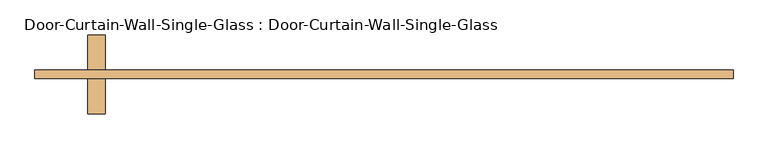
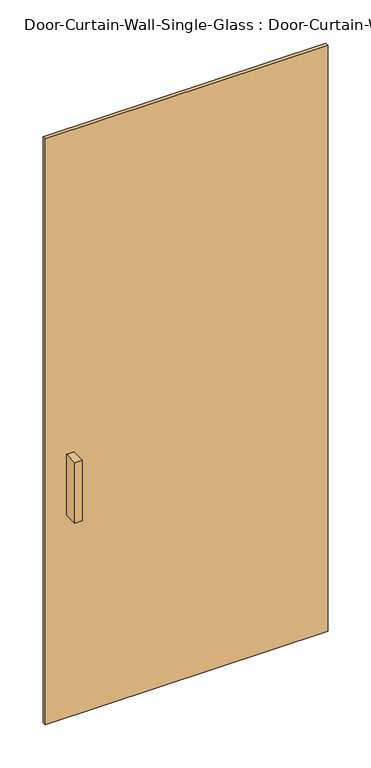
"""IFC4 building model written with IfcOpenShell, lengths in millimetres: door geometry, Door-Curtain-Wall-Single-Glass : Door-Curtain-Wall-Single-Glass."""

from ifc_helpers import new_model, si_unit, frame, origin, origin_with_axes, place, context, project, spatial, polyline, outline, extrude, source, transform, mapped, element, save


def door_curtain_wall_single_glass_door_curtain_wall_single_0bef0eec(model_context):
    return source(origin(), model_context, "Body", "SweptSolid", [
        extrude(outline(polyline([(503.3399533, -50.8), (-503.3399533, -50.8), (-503.3399533, -38.1), (503.3399533, -38.1), (503.3399533, -50.8)])), origin_with_axes(), (0.0, 0.0, 1.0), 2203.45),
        extrude(outline(polyline([(-401.7399533, 12.7), (-401.7399533, -38.1), (-427.1399533, -38.1), (-427.1399533, 12.7), (-401.7399533, 12.7)])), frame((0.0, 0.0, 762.0), z_axis=(0.0, 0.0, 1.0), x_axis=(1.0, 0.0, 0.0)), (0.0, 0.0, 1.0), 228.6),
        extrude(outline(polyline([(-427.1399533, -101.6), (-427.1399533, -50.8), (-401.7399533, -50.8), (-401.7399533, -101.6), (-427.1399533, -101.6)])), frame((0.0, 0.0, 762.0), z_axis=(0.0, 0.0, 1.0), x_axis=(1.0, 0.0, 0.0)), (0.0, 0.0, 1.0), 228.6),
    ])


if __name__ == "__main__":
    model = new_model("IFC4")
    model_context = context("Model", 3, world=origin())
    ifc_project = project(units=[si_unit("LENGTHUNIT", "METRE", prefix="MILLI")], contexts=[model_context])
    site = spatial("IfcSite", under=ifc_project)
    building = spatial("IfcBuilding", under=site)
    placement = place(None, origin())
    door_curtain_wall_single_glass_door_curtain_wall_single_shape = door_curtain_wall_single_glass_door_curtain_wall_single_0bef0eec(model_context)
    element("IfcDoor", 1, ObjectType="Door-Curtain-Wall-Single-Glass : Door-Curtain-Wall-Single-Glass", at=placement, inside=building, context=model_context, shape_type="MappedRepresentation", body=[
        mapped(door_curtain_wall_single_glass_door_curtain_wall_single_shape, transform((0.0, 0.0, 0.0), x_axis=(1.0, 0.0, 0.0), y_axis=(0.0, 1.0, 0.0), z_axis=(0.0, 0.0, 1.0))),
    ])
    save(model, "model.ifc")

# Revit data of these elements
# Type "Door-Curtain-Wall-Single-Glass : Door-Curtain-Wall-Single-Glass"
#   Type Mark = "EX"
#   Assembly Code = "B2030100"
#   Analytic Construction = "<None>"
#   Width [instance default] = 3' - 0"
#   Thermal Resistance (R) = 1.7611 (m²·K)/W
#   Swing Angle [instance default] = 90.00°
#   Heat Transfer Coefficient (U) = 0.567826 W/(m²·K)
#   Offset = 0' - 2"
#   Function = 1
#   Door Handle Material = Aluminum
#   Glazing = Glass
#   Visual Light Transmittance = 0
#   Solar Heat Gain Coefficient = 0
#   Construction Type Id = ""
# Element 1 (IfcDoor, "Door-Curtain-Wall-Single-Glass : Door-Curtain-Wall-Single-Glass")
#   Width = 3' - 3.63307"
#   Materials on its faces: "Aluminum", "Glass"
# Materials
#   "Aluminum": class "Metal", colour RGB 247 247 247, transparency 0, Description = "Aluminum 6061", Cost = 0
#   "Glass": class "Glass", colour RGB 218 227 224, transparency 0.85, Description = "Soda Lime Glass", Cost = 0
